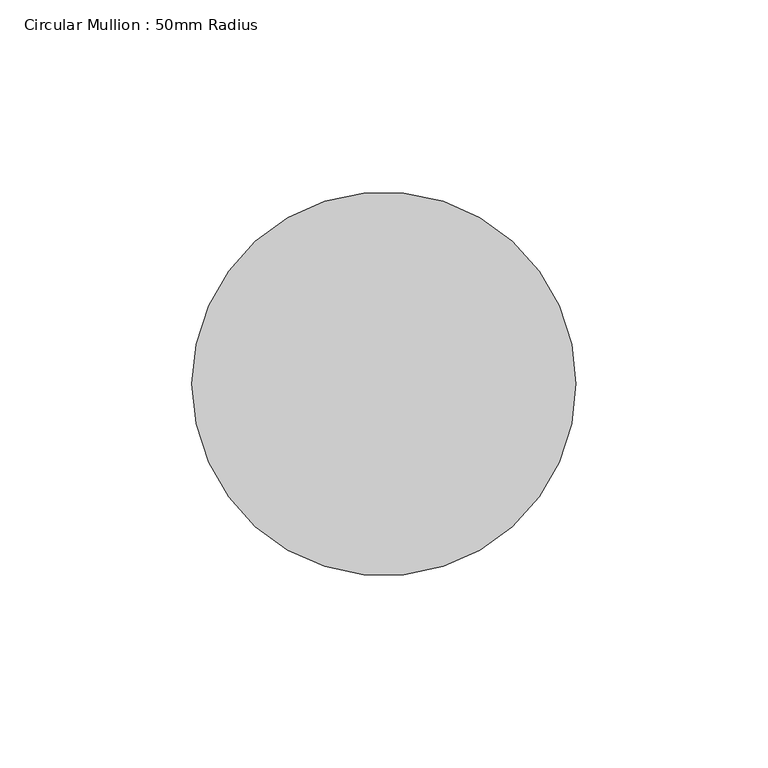
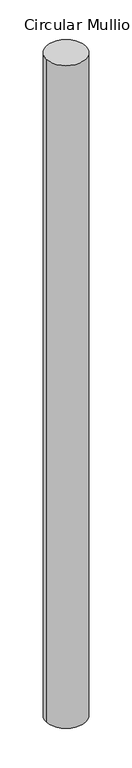
"""IFC4 building model written with IfcOpenShell, lengths in millimetres: member geometry, Circular Mullion : 50mm Radius."""

from ifc_helpers import new_model, si_unit, point, frame, frame_2d, origin, place, context, project, spatial, circle_curve, trimmed, segment, composite_curve, outline, extrude, source, transform, mapped, element, save


def circular_mullion_50mm_radius_d97d54af(model_context):
    return source(origin(), model_context, "Body", "SweptSolid", [
        extrude(outline(composite_curve([segment(trimmed(circle_curve(frame_2d((-50.0, 0.0)), 50.0), [point((0.0, 0.0))], [point((-100.0, 0.0))], False, "CARTESIAN"), True, "CONTINUOUS"), segment(trimmed(circle_curve(frame_2d((-50.0, 0.0)), 50.0), [point((-100.0, 0.0))], [point((0.0, 0.0))], False, "CARTESIAN"), True, "CONTINUOUS")], self_intersect=False)), frame((0.0, 0.0, -1779.4903986), z_axis=(0.0, 0.0, 1.0), x_axis=(1.0, 0.0, 0.0)), (0.0, 0.0, 1.0), 1779.4903986),
    ])


if __name__ == "__main__":
    model = new_model("IFC4")
    model_context = context("Model", 3, world=origin())
    ifc_project = project(units=[si_unit("LENGTHUNIT", "METRE", prefix="MILLI")], contexts=[model_context])
    site = spatial("IfcSite", under=ifc_project)
    building = spatial("IfcBuilding", under=site)
    placement = place(None, origin())
    circular_mullion_50mm_radius_shape = circular_mullion_50mm_radius_d97d54af(model_context)
    element("IfcMember", 1, ObjectType="Circular Mullion : 50mm Radius", at=placement, inside=building, context=model_context, shape_type="MappedRepresentation", body=[
        mapped(circular_mullion_50mm_radius_shape, transform((0.0, 0.0, 0.0), x_axis=(1.0, 0.0, 0.0), y_axis=(0.0, 1.0, 0.0), z_axis=(0.0, 0.0, 1.0))),
    ])
    save(model, "model.ifc")

# Revit data of these elements
# Type "Circular Mullion : 50mm Radius"
#   built-in parameter 1007350 = 0.164042 (stored number, unit not read)
# Element 1 (IfcMember, "Circular Mullion : 50mm Radius")
#   Materials on its faces: "Aluminium"
# Materials
#   "Aluminium": class "Metal", colour RGB 247 247 247, transparency 0, Description = "Aluminium 6061", Cost = 0
